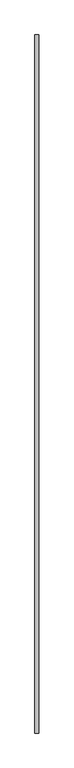
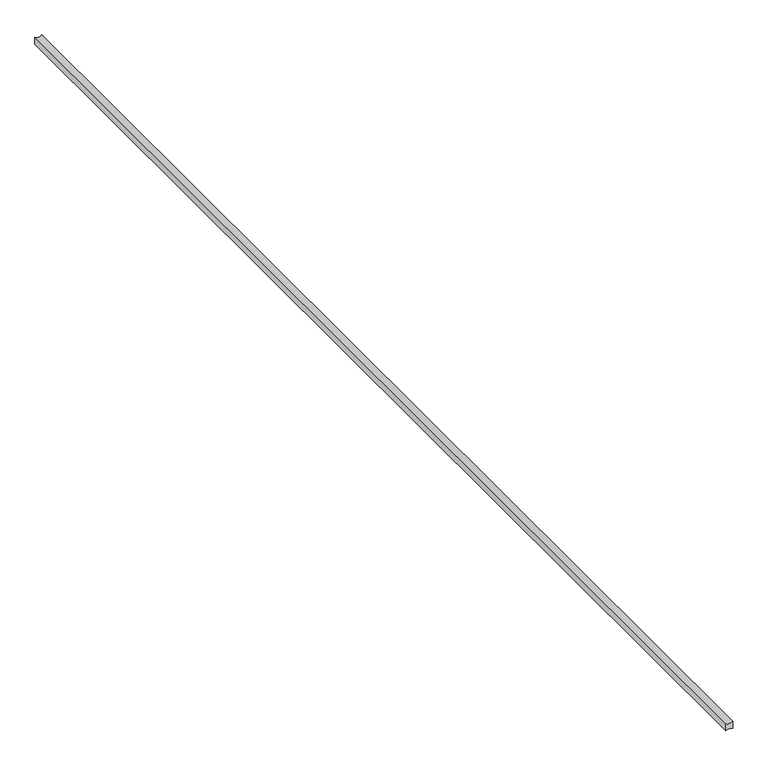
"""IFC4 building model written with IfcOpenShell, lengths in millimetres: proxy geometry, Joint047 7829 : Joint047 7829."""

from ifc_helpers import new_model, si_unit, point, frame, frame_2d, origin, place, context, project, spatial, polyline, circle_curve, trimmed, segment, composite_curve, outline, extrude, source, transform, mapped, element, save


def generic_models_cc2f93b6(model_context):
    return source(origin(), model_context, "Body", "SweptSolid", [
        extrude(outline(composite_curve([segment(polyline([(36569.4336936, -1990.9399414), (36582.096, -1990.9399414)]), True, "CONTINUOUS"), segment(trimmed(circle_curve(frame_2d((36587.1928449, -1996.6330454)), 7.6412866), [point((36582.096, -1990.9399414))], [point((36582.096, -2002.3261494))], True, "CARTESIAN"), True, "CONTINUOUS"), segment(polyline([(36582.096, -2002.3261494), (36569.4336936, -2002.3261494)]), True, "CONTINUOUS"), segment(trimmed(circle_curve(frame_2d((36560.506572, -1996.6330454)), 10.5879617), [point((36569.4336936, -2002.3261494))], [point((36569.4336936, -1990.9399414))], True, "CARTESIAN"), True, "CONTINUOUS")], self_intersect=False)), frame((0.0, 998.1570038, 0.0), z_axis=(0.0, 1.0, 0.0), x_axis=(0.0, 0.0, 1.0)), (0.0, 0.0, 1.0), 2000.0),
    ])


if __name__ == "__main__":
    model = new_model("IFC4")
    model_context = context("Model", 3, world=origin())
    ifc_project = project(units=[si_unit("LENGTHUNIT", "METRE", prefix="MILLI")], contexts=[model_context])
    site = spatial("IfcSite", under=ifc_project)
    building = spatial("IfcBuilding", under=site)
    placement = place(None, origin())
    generic_models_shape = generic_models_cc2f93b6(model_context)
    element("IfcBuildingElementProxy", 1, Name="Joint047 7829 : Joint047 7829", ObjectType="Joint047 7829 : Joint047 7829", at=placement, inside=building, context=model_context, shape_type="MappedRepresentation", body=[
        mapped(generic_models_shape, transform((0.0, 0.0, 0.0), x_axis=(1.0, 0.0, 0.0), y_axis=(0.0, 1.0, 0.0), z_axis=(0.0, 0.0, 1.0))),
    ])
    save(model, "model.ifc")

# Revit data of these elements
# Type "Joint047 7829 : Joint047 7829"
#   NameOverride = "Joint047"
# Element 1 (IfcBuildingElementProxy, "Joint047 7829 : Joint047 7829")
#   Materials on its faces: "SEALANT"
# Materials
#   "SEALANT": class "Unassigned", colour RGB 142 225 148, transparency 0
